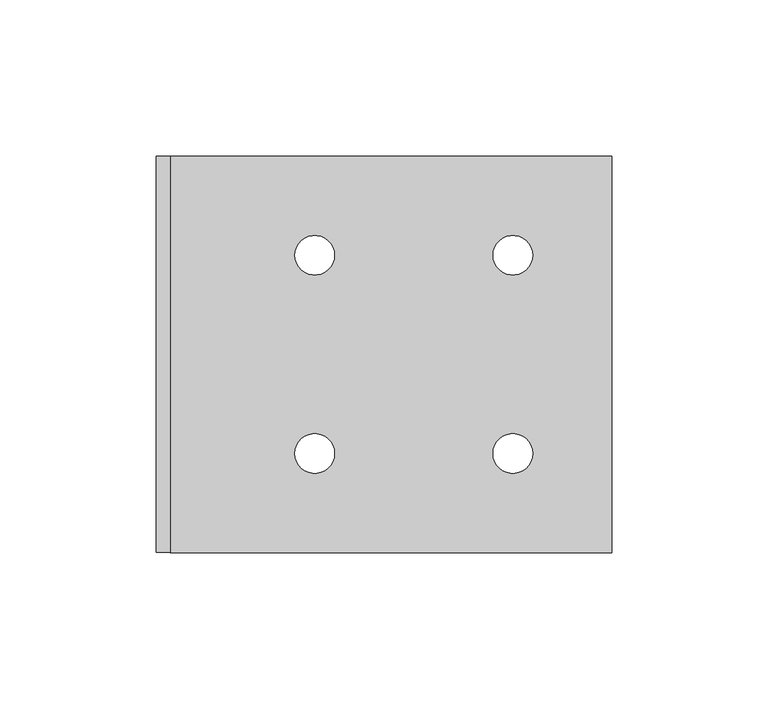
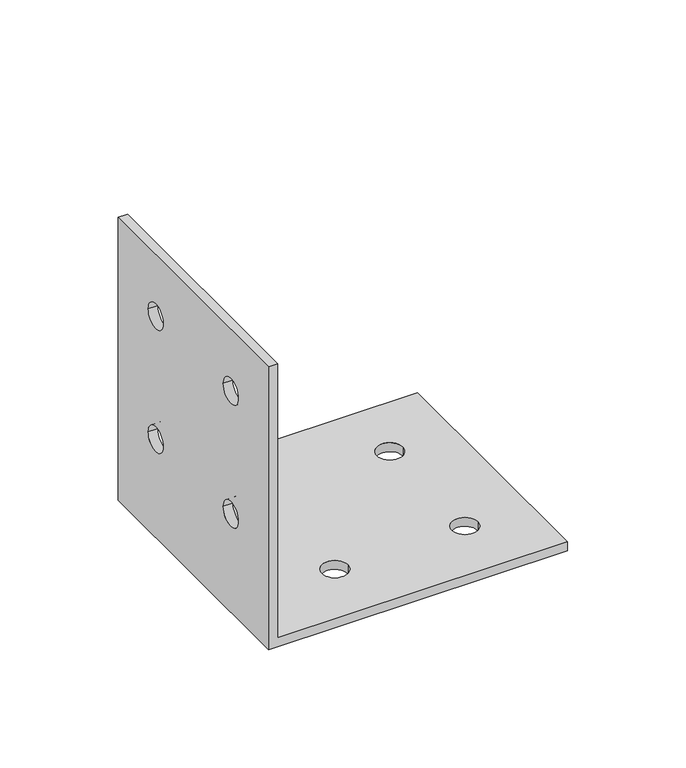
"""IFC4 building model written with IfcOpenShell, lengths in millimetres: fastener geometry."""

from ifc_helpers import new_model, si_unit, frame, origin, place, context, project, spatial, polyline, circle_curve, source, transform, mapped, element, save
from ifc_brep_helpers import plane_surface, revolved_surface, advanced_brep


def fastener_3f2cfda5(model_context):
    return source(origin(), model_context, "Body", "AdvancedBrep", [
        advanced_brep(
        [(4.5640625, -63.5, 146.05), (4.5640625, -63.5, 4.5640625), (4.5640625, 63.5, 4.5640625), (4.5640625, 63.5, 146.05), (4.5640625, 25.4, 50.8), (4.5640625, 38.1, 50.8), (4.5640625, -38.1, 50.8), (4.5640625, -25.4, 50.8), (4.5640625, -38.1, 114.3), (4.5640625, -25.4, 114.3), (4.5640625, 25.4, 114.3), (4.5640625, 38.1, 114.3), (0.0, 63.5, 146.05), (0.0, 63.5, 0.0), (0.0, -63.5, 0.0), (0.0, -63.5, 146.05), (0.0, 38.1, 50.8), (0.0, 25.4, 50.8), (0.0, -25.4, 50.8), (0.0, -38.1, 50.8), (0.0, -25.4, 114.3), (0.0, -38.1, 114.3), (0.0, 38.1, 114.3), (0.0, 25.4, 114.3), (146.05, 63.5, 4.5640625), (146.05, 63.5, 0.0), (146.05, -63.5, 0.0), (146.05, -63.5, 4.5640625), (57.15, 31.75, 4.5640625), (44.45, 31.75, 4.5640625), (120.65, 31.75, 4.5640625), (107.95, 31.75, 4.5640625), (57.15, -31.75, 4.5640625), (44.45, -31.75, 4.5640625), (120.65, -31.75, 4.5640625), (107.95, -31.75, 4.5640625), (44.45, 31.75, 0.0), (57.15, 31.75, 0.0), (107.95, 31.75, 0.0), (120.65, 31.75, 0.0), (44.45, -31.75, 0.0), (57.15, -31.75, 0.0), (107.95, -31.75, 0.0), (120.65, -31.75, 0.0)],
        [
            (0, 1),
            (1, 2),
            (2, 3),
            (3, 0),
            (4, 5, circle_curve(frame((4.5640625, 31.75, 50.8), z_axis=(-1.0, 0.0, 0.0), x_axis=(0.0, -1.0, 0.0)), 6.35)),
            (5, 4, circle_curve(frame((4.5640625, 31.75, 50.8), z_axis=(-1.0, 0.0, 0.0), x_axis=(0.0, -1.0, 0.0)), 6.35)),
            (6, 7, circle_curve(frame((4.5640625, -31.75, 50.8), z_axis=(-1.0, 0.0, 0.0), x_axis=(0.0, -1.0, 0.0)), 6.35)),
            (7, 6, circle_curve(frame((4.5640625, -31.75, 50.8), z_axis=(-1.0, 0.0, 0.0), x_axis=(0.0, -1.0, 0.0)), 6.35)),
            (8, 9, circle_curve(frame((4.5640625, -31.75, 114.3), z_axis=(-1.0, 0.0, 0.0), x_axis=(0.0, -1.0, 0.0)), 6.35)),
            (9, 8, circle_curve(frame((4.5640625, -31.75, 114.3), z_axis=(-1.0, 0.0, 0.0), x_axis=(0.0, -1.0, 0.0)), 6.35)),
            (10, 11, circle_curve(frame((4.5640625, 31.75, 114.3), z_axis=(-1.0, 0.0, 0.0), x_axis=(0.0, -1.0, 0.0)), 6.35)),
            (11, 10, circle_curve(frame((4.5640625, 31.75, 114.3), z_axis=(-1.0, 0.0, 0.0), x_axis=(0.0, -1.0, 0.0)), 6.35)),
            (12, 13),
            (13, 14),
            (14, 15),
            (15, 12),
            (16, 17, circle_curve(frame((0.0, 31.75, 50.8), z_axis=(1.0, 0.0, 0.0), x_axis=(0.0, -1.0, 0.0)), 6.35)),
            (17, 16, circle_curve(frame((0.0, 31.75, 50.8), z_axis=(1.0, 0.0, 0.0), x_axis=(0.0, -1.0, 0.0)), 6.35)),
            (18, 19, circle_curve(frame((0.0, -31.75, 50.8), z_axis=(1.0, 0.0, 0.0), x_axis=(0.0, -1.0, 0.0)), 6.35)),
            (19, 18, circle_curve(frame((0.0, -31.75, 50.8), z_axis=(1.0, 0.0, 0.0), x_axis=(0.0, -1.0, 0.0)), 6.35)),
            (20, 21, circle_curve(frame((0.0, -31.75, 114.3), z_axis=(1.0, 0.0, 0.0), x_axis=(0.0, -1.0, 0.0)), 6.35)),
            (21, 20, circle_curve(frame((0.0, -31.75, 114.3), z_axis=(1.0, 0.0, 0.0), x_axis=(0.0, -1.0, 0.0)), 6.35)),
            (22, 23, circle_curve(frame((0.0, 31.75, 114.3), z_axis=(1.0, 0.0, 0.0), x_axis=(0.0, -1.0, 0.0)), 6.35)),
            (23, 22, circle_curve(frame((0.0, 31.75, 114.3), z_axis=(1.0, 0.0, 0.0), x_axis=(0.0, -1.0, 0.0)), 6.35)),
            (3, 12),
            (15, 0),
            (2, 24),
            (24, 25),
            (25, 13),
            (14, 26),
            (26, 27),
            (27, 1),
            (27, 24),
            (28, 29, circle_curve(frame((50.8, 31.75, 4.5640625), z_axis=(0.0, 0.0, -1.0), x_axis=(1.0, 0.0, 0.0)), 6.35)),
            (29, 28, circle_curve(frame((50.8, 31.75, 4.5640625), z_axis=(0.0, 0.0, -1.0), x_axis=(1.0, 0.0, 0.0)), 6.35)),
            (30, 31, circle_curve(frame((114.3, 31.75, 4.5640625), z_axis=(0.0, 0.0, -1.0), x_axis=(1.0, 0.0, 0.0)), 6.35)),
            (31, 30, circle_curve(frame((114.3, 31.75, 4.5640625), z_axis=(0.0, 0.0, -1.0), x_axis=(1.0, 0.0, 0.0)), 6.35)),
            (32, 33, circle_curve(frame((50.8, -31.75, 4.5640625), z_axis=(0.0, 0.0, -1.0), x_axis=(1.0, 0.0, 0.0)), 6.35)),
            (33, 32, circle_curve(frame((50.8, -31.75, 4.5640625), z_axis=(0.0, 0.0, -1.0), x_axis=(1.0, 0.0, 0.0)), 6.35)),
            (34, 35, circle_curve(frame((114.3, -31.75, 4.5640625), z_axis=(0.0, 0.0, -1.0), x_axis=(1.0, 0.0, 0.0)), 6.35)),
            (35, 34, circle_curve(frame((114.3, -31.75, 4.5640625), z_axis=(0.0, 0.0, -1.0), x_axis=(1.0, 0.0, 0.0)), 6.35)),
            (25, 26),
            (36, 37, circle_curve(frame((50.8, 31.75, 0.0), z_axis=(0.0, 0.0, 1.0), x_axis=(1.0, 0.0, 0.0)), 6.35)),
            (37, 36, circle_curve(frame((50.8, 31.75, 0.0), z_axis=(0.0, 0.0, 1.0), x_axis=(1.0, 0.0, 0.0)), 6.35)),
            (38, 39, circle_curve(frame((114.3, 31.75, 0.0), z_axis=(0.0, 0.0, 1.0), x_axis=(1.0, 0.0, 0.0)), 6.35)),
            (39, 38, circle_curve(frame((114.3, 31.75, 0.0), z_axis=(0.0, 0.0, 1.0), x_axis=(1.0, 0.0, 0.0)), 6.35)),
            (40, 41, circle_curve(frame((50.8, -31.75, 0.0), z_axis=(0.0, 0.0, 1.0), x_axis=(1.0, 0.0, 0.0)), 6.35)),
            (41, 40, circle_curve(frame((50.8, -31.75, 0.0), z_axis=(0.0, 0.0, 1.0), x_axis=(1.0, 0.0, 0.0)), 6.35)),
            (42, 43, circle_curve(frame((114.3, -31.75, 0.0), z_axis=(0.0, 0.0, 1.0), x_axis=(1.0, 0.0, 0.0)), 6.35)),
            (43, 42, circle_curve(frame((114.3, -31.75, 0.0), z_axis=(0.0, 0.0, 1.0), x_axis=(1.0, 0.0, 0.0)), 6.35)),
            (29, 36),
            (37, 28),
            (39, 30),
            (31, 38),
            (41, 32),
            (33, 40),
            (43, 34),
            (35, 42),
            (5, 16),
            (17, 4),
            (19, 6),
            (7, 18),
            (21, 8),
            (9, 20),
            (23, 10),
            (11, 22),
        ],
        [
            plane_surface(frame((4.5640625, 63.5, 146.05), z_axis=(1.0, 0.0, 0.0), x_axis=(0.0, 1.0, 0.0))),
            plane_surface(frame((0.0, 63.5, 146.05), z_axis=(-1.0, 0.0, 0.0), x_axis=(0.0, -1.0, 0.0))),
            plane_surface(frame((4.5640625, -63.5, 146.05), z_axis=(0.0, 0.0, 1.0), x_axis=(-1.0, 0.0, 0.0))),
            plane_surface(frame((4.5640625, 63.5, 146.05), z_axis=(0.0, 1.0, 0.0), x_axis=(-1.0, 0.0, 0.0))),
            plane_surface(frame((4.5640625, -63.5, 4.5640625), z_axis=(0.0, -1.0, 0.0), x_axis=(-1.0, 0.0, 0.0))),
            plane_surface(frame((0.0, -63.5, 4.5640625), z_axis=(0.0, 0.0, 1.0), x_axis=(-1.0, 0.0, 0.0))),
            plane_surface(frame((0.0, -63.5, 0.0), z_axis=(0.0, 0.0, -1.0), x_axis=(1.0, 0.0, 0.0))),
            plane_surface(frame((146.05, 63.5, 4.5640625), z_axis=(1.0, 0.0, 0.0), x_axis=(0.0, 0.0, -1.0))),
            revolved_surface(polyline([(57.15, 31.75, 4.5640625), (57.15, 31.75, 0.0)]), (50.8, 31.75, 0.0), (0.0, 0.0, 1.0)),
            revolved_surface(polyline([(120.64999999999999, 31.75, 4.5640625), (120.64999999999999, 31.75, 0.0)]), (114.3, 31.75, 0.0), (0.0, 0.0, 1.0)),
            revolved_surface(polyline([(57.15, -31.75, 4.5640625), (57.15, -31.75, 0.0)]), (50.8, -31.75, 0.0), (0.0, 0.0, 1.0)),
            revolved_surface(polyline([(120.64999999999999, -31.75, 4.5640625), (120.64999999999999, -31.75, 0.0)]), (114.3, -31.75, 0.0), (0.0, 0.0, 1.0)),
            revolved_surface(polyline([(4.5640625, 25.4, 50.8), (0.0, 25.4, 50.8)]), (0.0, 31.75, 50.8), (1.0, 0.0, 0.0)),
            revolved_surface(polyline([(4.5640625, -38.1, 50.8), (0.0, -38.1, 50.8)]), (0.0, -31.75, 50.8), (1.0, 0.0, 0.0)),
            revolved_surface(polyline([(4.5640625, -38.1, 114.3), (0.0, -38.1, 114.3)]), (0.0, -31.75, 114.3), (1.0, 0.0, 0.0)),
            revolved_surface(polyline([(4.5640625, 25.4, 114.3), (0.0, 25.4, 114.3)]), (0.0, 31.75, 114.3), (1.0, 0.0, 0.0)),
        ],
        [
            (0, [[1, 2, 3, 4], [5, 6], [7, 8], [9, 10], [11, 12]]),
            (1, [[13, 14, 15, 16], [17, 18], [19, 20], [21, 22], [23, 24]]),
            (2, [[25, -16, 26, -4]]),
            (3, [[27, 28, 29, -13, -25, -3]]),
            (4, [[-26, -15, 30, 31, 32, -1]]),
            (5, [[-27, -2, -32, 33], [34, 35], [36, 37], [38, 39], [40, 41]]),
            (6, [[-30, -14, -29, 42], [43, 44], [45, 46], [47, 48], [49, 50]]),
            (7, [[-31, -42, -28, -33]]),
            (8, [[-35, 51, -44, 52]]),
            (8, [[-43, -51, -34, -52]]),
            (9, [[-46, 53, -37, 54]]),
            (9, [[-36, -53, -45, -54]]),
            (10, [[-48, 55, -39, 56]]),
            (10, [[-38, -55, -47, -56]]),
            (11, [[-50, 57, -41, 58]]),
            (11, [[-40, -57, -49, -58]]),
            (12, [[-6, 59, -18, 60]]),
            (12, [[-17, -59, -5, -60]]),
            (13, [[-20, 61, -8, 62]]),
            (13, [[-7, -61, -19, -62]]),
            (14, [[-22, 63, -10, 64]]),
            (14, [[-9, -63, -21, -64]]),
            (15, [[-24, 65, -12, 66]]),
            (15, [[-11, -65, -23, -66]]),
        ],
    ),
    ])


if __name__ == "__main__":
    model = new_model("IFC4")
    model_context = context("Model", 3, world=origin())
    ifc_project = project(units=[si_unit("LENGTHUNIT", "METRE", prefix="MILLI")], contexts=[model_context])
    site = spatial("IfcSite", under=ifc_project)
    building = spatial("IfcBuilding", under=site)
    placement = place(None, origin())
    fastener_shape = fastener_3f2cfda5(model_context)
    element("IfcFastener", 1, ObjectType="060523 - W_P_C - Fastenings - Simpson - HLGPC Heavy Angles and Gussets NO BOLTS : SIMPSON -HL55 - 5 X 5.75 - .5\" BOLT - HDG", at=placement, inside=building, context=model_context, shape_type="MappedRepresentation", body=[
        mapped(fastener_shape, transform((0.0, 0.0, 0.0), x_axis=(1.0, 0.0, 0.0), y_axis=(0.0, 1.0, 0.0), z_axis=(0.0, 0.0, 1.0))),
    ])
    save(model, "model.ifc")

# Revit data of these elements
# Type "060523 - W_P_C - Fastenings - Simpson - HLGPC Heavy Angles and Gussets NO BOLTS : SIMPSON -HL55 - 5 X 5.75 - .5\" BOLT - HDG"
#   URL = "https://www.strongtie.com/classiccollection_architecturalproductsgroup/hlpc-hlgpc_productgroup_wcc/p/hlpc.hlgpc"
#   L = 0' - 5"
#   Hole Radius = 0' - 0 1/4"
#   D4 = 0' - 2 1/2"
#   D2 = 0' - 2 1/2"
#   D1 = 0' - 1 1/4"
#   D3 = 0' - 2"
#   Ga. = 0' - 0 23/128"
#   W1 & W2 = 0' - 5 3/4"
#   Default Elevation = 4' - 0"
#   Bolt Visibility - 3B = no
#   Bolt Visibility - 3A = no
#   Bolt Visibility - 2B = yes
#   Bolt Visibility - 2A = yes
#   Bolt Visibility - 1B = yes
#   Bolt Visibility - 1A = yes
#   Bolt Visibility = yes
#   Bolt Size = element 1549524
# Element 1 (IfcFastener, "060523 - W_P_C - Fastenings - Simpson - HLGPC Heavy Angles and Gussets NO BOLTS : SIMPSON -HL55 - 5 X 5.75 - .5\" BOLT - HDG")
#   Materials on its faces: "SIMPSON -HL55 - 5 X 5.75 - .5\" BOLT (3 GA - RAW STEEL - NO FINISH)"
# Materials
#   "SIMPSON -HL55 - 5 X 5.75 - .5\" BOLT (3 GA - RAW STEEL - NO FINISH)": class "Generic", colour RGB 120 120 120, transparency 0, Cost = 0
